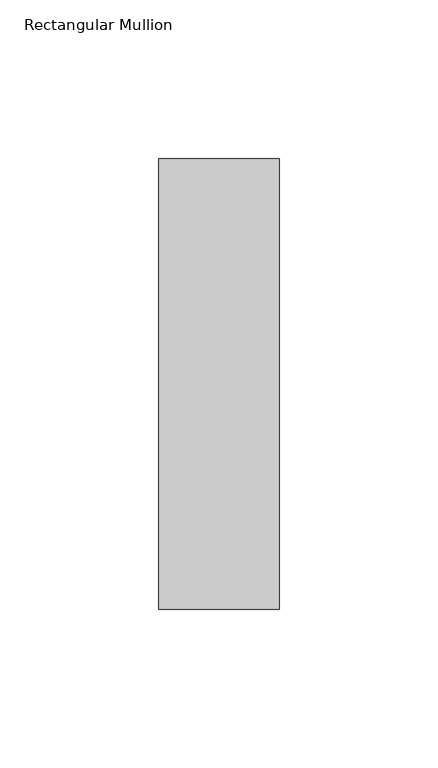
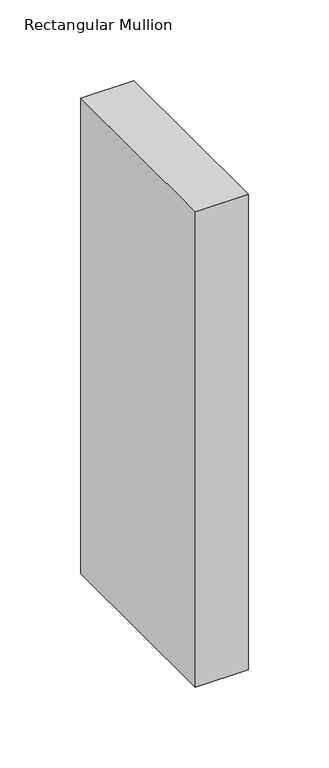
"""IFC4 building model written with IfcOpenShell, lengths in millimetres: member geometry, Rectangular Mullion : NLRS_21_CWM_hsb-regel 38x142_gen_rsf."""

import ifcopenshell
import ifcopenshell.guid

model = None  # the IFC model being written
_history = None  # IfcOwnerHistory: only IFC2X3 demands one
_inside = {}  # id of a spatial element -> (the spatial element, [elements in it])
_under = {}  # id of a project, library or spatial element -> (it, [spatial elements below it])
_declared = {}  # id of a project -> (the project, [libraries it declares])
_typed = {}  # id of a type object -> (the type object, [elements of that type])
_made_of = {}  # id of a material, layer set ... -> (it, [elements and type objects made of it])


def new_model(schema):
    """Start an empty IFC model of exactly this schema.

    Asked for "IFC4X3", IfcOpenShell would pick the latest addendum, in which some entities
    have other attributes; the version numbers below select the first issue.
    IFC2X3 requires an IfcOwnerHistory on every rooted entity: one is made here for all.
    """
    global model, _history
    if schema == "IFC4X3":
        model = ifcopenshell.file(schema_version=(4, 3, 0, 0))
    else:
        model = ifcopenshell.file(schema=schema)
    _inside.clear()
    _under.clear()
    _declared.clear()
    _typed.clear()
    _made_of.clear()
    _history = None
    if model.schema == "IFC2X3":
        org = make("IfcOrganization", Name="unknown")
        user = make(
            "IfcPersonAndOrganization",
            ThePerson=make("IfcPerson", FamilyName="unknown"),
            TheOrganization=org,
        )
        app = make(
            "IfcApplication",
            ApplicationDeveloper=org,
            Version="unknown",
            ApplicationFullName="unknown",
            ApplicationIdentifier="unknown",
        )
        _history = make(
            "IfcOwnerHistory",
            OwningUser=user,
            OwningApplication=app,
            ChangeAction="ADDED",
            CreationDate=0,
        )
    return model


def make(cls, **values):
    """One entity of the class cls with the attributes given. An attribute that is None is left unset."""
    return model.create_entity(
        cls, **{name: value for name, value in values.items() if value is not None}
    )


def rooted(cls, **values):
    """An entity with a GlobalId (a new one), such as an element, a storey or a relation."""
    return make(cls, GlobalId=ifcopenshell.guid.new(), OwnerHistory=_history, **values)


def si_unit(unit_type, name, prefix=None):
    """IfcSIUnit, for example si_unit("LENGTHUNIT", "METRE", prefix="MILLI")."""
    return make("IfcSIUnit", UnitType=unit_type, Prefix=prefix, Name=name)


def assignment(units):
    """IfcUnitAssignment: the units of a project."""
    return None if units is None else make("IfcUnitAssignment", Units=units)


def point(xyz):
    """IfcCartesianPoint."""
    return None if xyz is None else make("IfcCartesianPoint", Coordinates=xyz)


def direction(xyz):
    """IfcDirection."""
    return None if xyz is None else make("IfcDirection", DirectionRatios=xyz)


def frame(location, z_axis=None, x_axis=None):
    """IfcAxis2Placement3D, a coordinate frame: its origin and axes. An axis left out is left unset."""
    return make(
        "IfcAxis2Placement3D",
        Location=point(location),
        Axis=direction(z_axis),
        RefDirection=direction(x_axis),
    )


def origin():
    """The frame at (0, 0, 0) with its axes left unset."""
    return frame((0.0, 0.0, 0.0))


def place(relative_to, where):
    """IfcLocalPlacement: puts the frame where relative to a parent placement (None: the world)."""
    return make(
        "IfcLocalPlacement", PlacementRelTo=relative_to, RelativePlacement=where
    )


def context(
    kind, dimensions, precision=None, world=None, true_north=None, identifier=None
):
    """IfcGeometricRepresentationContext, for example the 3D "Model" context."""
    return make(
        "IfcGeometricRepresentationContext",
        ContextIdentifier=identifier,
        ContextType=kind,
        CoordinateSpaceDimension=dimensions,
        Precision=precision,
        WorldCoordinateSystem=world,
        TrueNorth=true_north,
    )


def project(units=None, contexts=None):
    """IfcProject with its units and contexts."""
    return rooted(
        "IfcProject",
        Name="project",
        RepresentationContexts=contexts,
        UnitsInContext=assignment(units),
    )


def spatial(cls, under=None, at=None, **own):
    """A site, building, storey or space (cls), placed at a placement, below another one or the project."""
    s = rooted(cls, ObjectPlacement=at, **own)
    if under is not None:
        _under.setdefault(under.id(), (under, []))[1].append(s)
    return s


def polyline(points):
    """IfcPolyline through the points."""
    return make("IfcPolyline", Points=[point(p) for p in points])


def outline(outer, holes=None, kind="AREA"):
    """IfcArbitraryClosedProfileDef: a profile drawn as a closed curve; with holes, ...WithVoids."""
    if holes is None:
        return make("IfcArbitraryClosedProfileDef", ProfileType=kind, OuterCurve=outer)
    return make(
        "IfcArbitraryProfileDefWithVoids",
        ProfileType=kind,
        OuterCurve=outer,
        InnerCurves=holes,
    )


def extrude(swept, where, along, depth):
    """IfcExtrudedAreaSolid: the profile swept, set in the frame where, extruded along a direction by depth."""
    return make(
        "IfcExtrudedAreaSolid",
        SweptArea=swept,
        Position=where,
        ExtrudedDirection=direction(along),
        Depth=depth,
    )


def shape(context_of_items, identifier, shape_type, items):
    """IfcShapeRepresentation: the items that make up one representation, for example the "Body"."""
    return make(
        "IfcShapeRepresentation",
        ContextOfItems=context_of_items,
        RepresentationIdentifier=identifier,
        RepresentationType=shape_type,
        Items=items,
    )


def source(mapping_origin, context_of_items, identifier, shape_type, items):
    """IfcRepresentationMap: a shape defined once, which mapped items show again and again."""
    return make(
        "IfcRepresentationMap",
        MappingOrigin=mapping_origin,
        MappedRepresentation=shape(context_of_items, identifier, shape_type, items),
    )


def transform(
    local_origin,
    x_axis=None,
    y_axis=None,
    z_axis=None,
    scale=None,
    scale2=None,
    scale3=None,
    uniform=True,
):
    """IfcCartesianTransformationOperator3D, or its non-uniform kind. x_axis, y_axis, z_axis: its Axis1, 2, 3."""
    if uniform:
        return make(
            "IfcCartesianTransformationOperator3D",
            Axis1=direction(x_axis),
            Axis2=direction(y_axis),
            LocalOrigin=point(local_origin),
            Scale=scale,
            Axis3=direction(z_axis),
        )
    return make(
        "IfcCartesianTransformationOperator3DnonUniform",
        Axis1=direction(x_axis),
        Axis2=direction(y_axis),
        LocalOrigin=point(local_origin),
        Scale=scale,
        Axis3=direction(z_axis),
        Scale2=scale2,
        Scale3=scale3,
    )


def mapped(mapping_source, mapping_target):
    """IfcMappedItem: shows the shape of a source again, moved by a transform."""
    return make(
        "IfcMappedItem", MappingSource=mapping_source, MappingTarget=mapping_target
    )


def made_of(thing, what):
    """Note that an element or type object is made of a material, layer set ...; save() writes the relation."""
    if what is not None:
        _made_of.setdefault(what.id(), (what, []))[1].append(thing)
    return thing


def element(
    cls,
    number,
    at=None,
    inside=None,
    cuts=None,
    type_object=None,
    material=None,
    context=None,
    identifier="Body",
    shape_type=None,
    held_by="IfcProductDefinitionShape",
    body=None,
    shapes=None,
    **own,
):
    """One element of the class cls, such as IfcWall. Its Tag is "e" and its number.

    at: its placement. inside: the storey or other place that contains it. cuts: it is an
    opening in that element (IfcRelVoidsElement). A single representation is given by context,
    identifier, shape_type and body (its items); several are given by shapes. held_by: the class
    of the entity that holds the representations. save() writes the other relations.
    """
    e = rooted(cls, Tag="e%d" % number, ObjectPlacement=at, **own)
    if body is not None:
        shapes = [shape(context, identifier, shape_type, body)]
    if shapes is not None:
        e.Representation = make(held_by, Representations=shapes)
    if inside is not None:
        _inside.setdefault(inside.id(), (inside, []))[1].append(e)
    if cuts is not None:
        rooted(
            "IfcRelVoidsElement", RelatingBuildingElement=cuts, RelatedOpeningElement=e
        )
    if type_object is not None:
        _typed.setdefault(type_object.id(), (type_object, []))[1].append(e)
    return made_of(e, material)


def aggregate(whole, parts):
    """IfcRelAggregates: a whole, such as a stair, and the parts it consists of."""
    return rooted("IfcRelAggregates", RelatingObject=whole, RelatedObjects=parts)


def save(model, path):
    """Write the relations noted so far, then the file.

    IfcRelAggregates (storeys below a building ...), IfcRelContainedInSpatialStructure (elements
    in a storey), IfcRelDefinesByType, IfcRelAssociatesMaterial and IfcRelDeclares: one each for
    every whole, place, type object, material and project.
    """
    for whole, parts in _under.values():
        aggregate(whole, parts)
    for where, things in _inside.values():
        rooted(
            "IfcRelContainedInSpatialStructure",
            RelatedElements=things,
            RelatingStructure=where,
        )
    for kind, things in _typed.values():
        rooted("IfcRelDefinesByType", RelatedObjects=things, RelatingType=kind)
    for what, things in _made_of.values():
        rooted("IfcRelAssociatesMaterial", RelatedObjects=things, RelatingMaterial=what)
    for by, libraries in _declared.values():
        rooted("IfcRelDeclares", RelatingContext=by, RelatedDefinitions=libraries)
    model.write(path)


def rectangular_mullion_ee68c600(model_context):
    return source(origin(), model_context, "Body", "SweptSolid", [
        extrude(outline(polyline([(-38.0, -71.0), (-38.0, 71.0), (0.0, 71.0), (0.0, -71.0), (-38.0, -71.0)])), frame((0.0, 0.0, -359.9999997), z_axis=(0.0, 0.0, 1.0), x_axis=(1.0, 0.0, 0.0)), (0.0, 0.0, 1.0), 359.9999997),
    ])


if __name__ == "__main__":
    model = new_model("IFC4")
    model_context = context("Model", 3, world=origin())
    ifc_project = project(units=[si_unit("LENGTHUNIT", "METRE", prefix="MILLI")], contexts=[model_context])
    site = spatial("IfcSite", under=ifc_project)
    building = spatial("IfcBuilding", under=site)
    placement = place(None, origin())
    rectangular_mullion_shape = rectangular_mullion_ee68c600(model_context)
    element("IfcMember", 1, ObjectType="Rectangular Mullion : NLRS_21_CWM_hsb-regel 38x142_gen_rsf", at=placement, inside=building, context=model_context, shape_type="MappedRepresentation", body=[
        mapped(rectangular_mullion_shape, transform((0.0, 0.0, 0.0), x_axis=(1.0, 0.0, 0.0), y_axis=(0.0, 1.0, 0.0), z_axis=(0.0, 0.0, 1.0))),
    ])
    save(model, "model.ifc")

# Revit data of these elements
# Type "Rectangular Mullion : NLRS_21_CWM_hsb-regel 38x142_gen_rsf"
#   Export Type to IFC As = "IfcWall"
#   Type IfcGUID = "07M7mRoiH1CR8m_RSKIwpF"
#   Assembly Code = "21.10"
#   built-in parameter 1007322 = 0.465879 (stored number, unit not read)
#   built-in parameter 1007321 = 0.062336 (stored number, unit not read)
#   built-in parameter 1007320 = 0.062336 (stored number, unit not read)
# Element 1 (IfcMember, "Rectangular Mullion : NLRS_21_CWM_hsb-regel 38x142_gen_rsf")
#   Materials on its faces: "NLRS_i2_hout naaldhout vuren_gen_rsf"
# Materials
#   "NLRS_i2_hout naaldhout vuren_gen_rsf": class "I - Hout", colour RGB 234 199 147, transparency 0, Keynote = "i2", Manufacturer = "Revit Standards Foundation", URL = "www.revitstandards.org", Description = "hout vuren", Cost = 0
